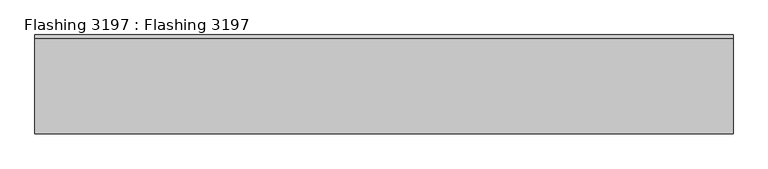
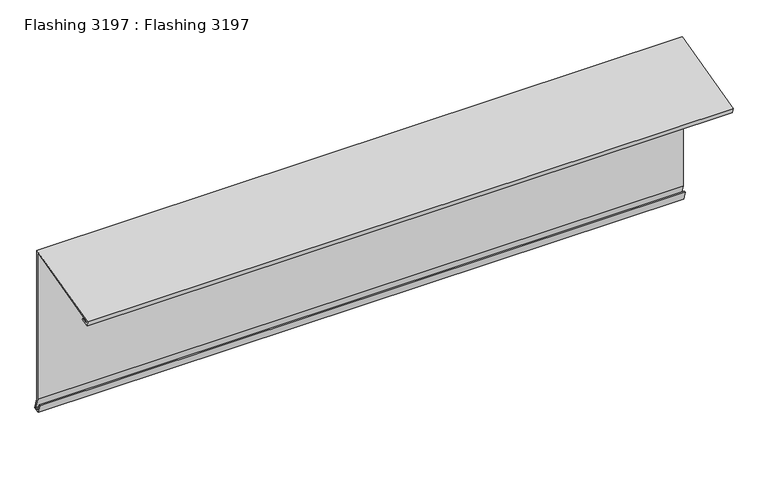
"""IFC4 building model written with IfcOpenShell, lengths in millimetres: proxy geometry, Flashing 3197 : Flashing 3197."""

from ifc_helpers import new_model, si_unit, frame, origin, place, context, project, spatial, polyline, outline, extrude, source, transform, mapped, element, save


def flashing_3197_flashing_3197_086f2f6e(model_context):
    return source(origin(), model_context, "Body", "SweptSolid", [
        extrude(outline(polyline([(10550.3613281, 43920.3046875), (10546.9589844, 43935.2734375), (10819.5097656, 44004.90625), (10819.5097656, 43518.7539063), (10830.6904297, 43482.3320313), (10813.1210937, 43476.9648438), (10804.5996094, 43504.4882813), (10808.4206617, 43505.6713107), (10815.7635636, 43481.9545626), (10825.6911014, 43484.9872871), (10815.5097656, 43518.1537731), (10815.5097656, 43999.7558251), (10551.7227627, 43932.3620321), (10553.3654045, 43925.1351625), (10575.0634961, 43930.3201524), (10575.9931641, 43926.4296875), (10550.3613281, 43920.3046875)])), frame((3694.0383192, 0.0, 0.0), z_axis=(1.0, 0.0, 0.0), x_axis=(0.0, 1.0, 0.0)), (0.0, 0.0, 1.0), 2000.25),
    ])


if __name__ == "__main__":
    model = new_model("IFC4")
    model_context = context("Model", 3, world=origin())
    ifc_project = project(units=[si_unit("LENGTHUNIT", "METRE", prefix="MILLI")], contexts=[model_context])
    site = spatial("IfcSite", under=ifc_project)
    building = spatial("IfcBuilding", under=site)
    placement = place(None, origin())
    flashing_3197_flashing_3197_shape = flashing_3197_flashing_3197_086f2f6e(model_context)
    element("IfcBuildingElementProxy", 1, Name="Flashing 3197 : Flashing 3197", ObjectType="Flashing 3197 : Flashing 3197", at=placement, inside=building, context=model_context, shape_type="MappedRepresentation", body=[
        mapped(flashing_3197_flashing_3197_shape, transform((0.0, 0.0, 0.0), x_axis=(1.0, 0.0, 0.0), y_axis=(0.0, 1.0, 0.0), z_axis=(0.0, 0.0, 1.0))),
    ])
    save(model, "model.ifc")

# Revit data of these elements
# Type "Flashing 3197 : Flashing 3197"
#   NameOverride = "Flashing"
# Element 1 (IfcBuildingElementProxy, "Flashing 3197 : Flashing 3197")
#   Materials on its faces: "HIGH EAVE FLASHING"
# Materials
#   "HIGH EAVE FLASHING": class "Unassigned", colour RGB 128 128 128, transparency 0
